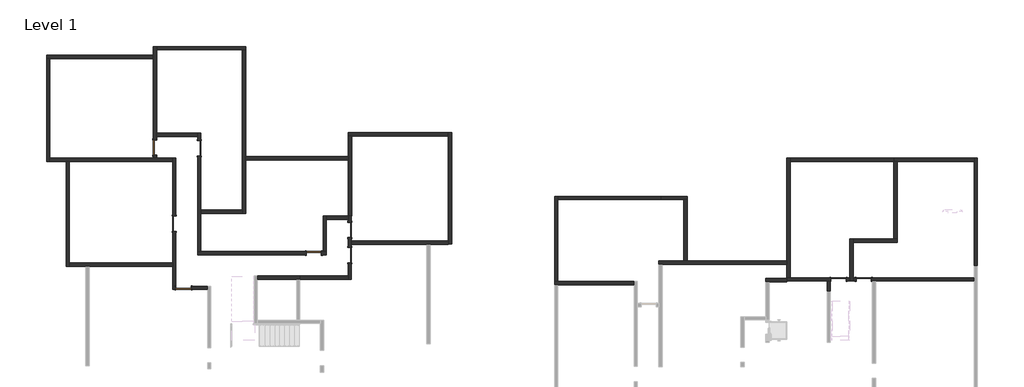
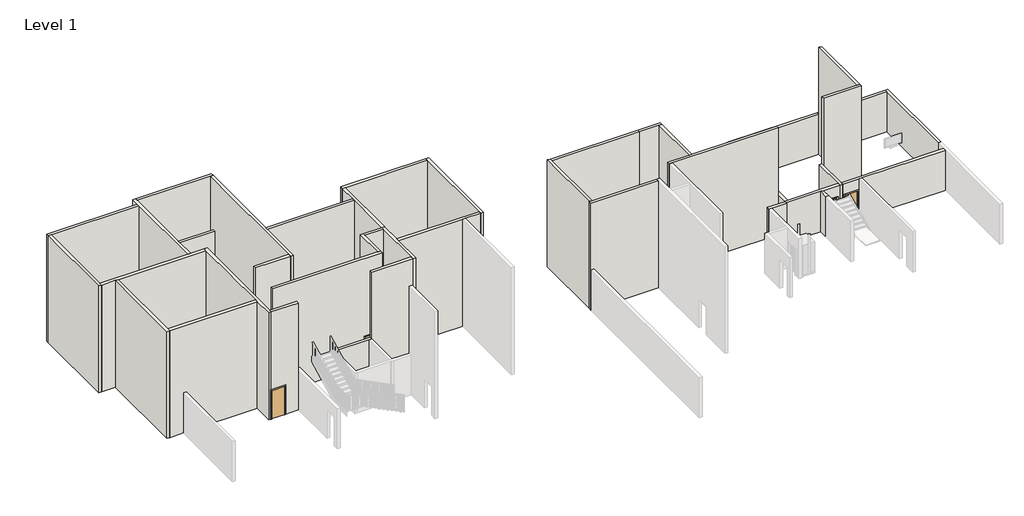
# One storey, part 2 of 3: 41 walls, 9 doors.
"""IFC4 building model written with IfcOpenShell, lengths in millimetres."""

import ifcopenshell
import ifcopenshell.guid

model = None  # the IFC model being written
_history = None  # IfcOwnerHistory: only IFC2X3 demands one
_inside = {}  # id of a spatial element -> (the spatial element, [elements in it])
_under = {}  # id of a project, library or spatial element -> (it, [spatial elements below it])
_declared = {}  # id of a project -> (the project, [libraries it declares])
_typed = {}  # id of a type object -> (the type object, [elements of that type])
_made_of = {}  # id of a material, layer set ... -> (it, [elements and type objects made of it])


def new_model(schema):
    """Start an empty IFC model of exactly this schema.

    Asked for "IFC4X3", IfcOpenShell would pick the latest addendum, in which some entities
    have other attributes; the version numbers below select the first issue.
    IFC2X3 requires an IfcOwnerHistory on every rooted entity: one is made here for all.
    """
    global model, _history
    if schema == "IFC4X3":
        model = ifcopenshell.file(schema_version=(4, 3, 0, 0))
    else:
        model = ifcopenshell.file(schema=schema)
    _inside.clear()
    _under.clear()
    _declared.clear()
    _typed.clear()
    _made_of.clear()
    _history = None
    if model.schema == "IFC2X3":
        org = make("IfcOrganization", Name="unknown")
        user = make(
            "IfcPersonAndOrganization",
            ThePerson=make("IfcPerson", FamilyName="unknown"),
            TheOrganization=org,
        )
        app = make(
            "IfcApplication",
            ApplicationDeveloper=org,
            Version="unknown",
            ApplicationFullName="unknown",
            ApplicationIdentifier="unknown",
        )
        _history = make(
            "IfcOwnerHistory",
            OwningUser=user,
            OwningApplication=app,
            ChangeAction="ADDED",
            CreationDate=0,
        )
    return model


def make(cls, **values):
    """One entity of the class cls with the attributes given. An attribute that is None is left unset."""
    return model.create_entity(
        cls, **{name: value for name, value in values.items() if value is not None}
    )


def rooted(cls, **values):
    """An entity with a GlobalId (a new one), such as an element, a storey or a relation."""
    return make(cls, GlobalId=ifcopenshell.guid.new(), OwnerHistory=_history, **values)


def si_unit(unit_type, name, prefix=None):
    """IfcSIUnit, for example si_unit("LENGTHUNIT", "METRE", prefix="MILLI")."""
    return make("IfcSIUnit", UnitType=unit_type, Prefix=prefix, Name=name)


def assignment(units):
    """IfcUnitAssignment: the units of a project."""
    return None if units is None else make("IfcUnitAssignment", Units=units)


def point(xyz):
    """IfcCartesianPoint."""
    return None if xyz is None else make("IfcCartesianPoint", Coordinates=xyz)


def direction(xyz):
    """IfcDirection."""
    return None if xyz is None else make("IfcDirection", DirectionRatios=xyz)


def frame(location, z_axis=None, x_axis=None):
    """IfcAxis2Placement3D, a coordinate frame: its origin and axes. An axis left out is left unset."""
    return make(
        "IfcAxis2Placement3D",
        Location=point(location),
        Axis=direction(z_axis),
        RefDirection=direction(x_axis),
    )


def origin():
    """The frame at (0, 0, 0) with its axes left unset."""
    return frame((0.0, 0.0, 0.0))


def origin_with_axes():
    """The frame at (0, 0, 0) with the z axis (0, 0, 1) and the x axis (1, 0, 0) written out."""
    return frame((0.0, 0.0, 0.0), z_axis=(0.0, 0.0, 1.0), x_axis=(1.0, 0.0, 0.0))


def place(relative_to, where):
    """IfcLocalPlacement: puts the frame where relative to a parent placement (None: the world)."""
    return make(
        "IfcLocalPlacement", PlacementRelTo=relative_to, RelativePlacement=where
    )


def context(
    kind, dimensions, precision=None, world=None, true_north=None, identifier=None
):
    """IfcGeometricRepresentationContext, for example the 3D "Model" context."""
    return make(
        "IfcGeometricRepresentationContext",
        ContextIdentifier=identifier,
        ContextType=kind,
        CoordinateSpaceDimension=dimensions,
        Precision=precision,
        WorldCoordinateSystem=world,
        TrueNorth=true_north,
    )


def project(units=None, contexts=None):
    """IfcProject with its units and contexts."""
    return rooted(
        "IfcProject",
        Name="project",
        RepresentationContexts=contexts,
        UnitsInContext=assignment(units),
    )


def spatial(cls, under=None, at=None, **own):
    """A site, building, storey or space (cls), placed at a placement, below another one or the project."""
    s = rooted(cls, ObjectPlacement=at, **own)
    if under is not None:
        _under.setdefault(under.id(), (under, []))[1].append(s)
    return s


def polyline(points):
    """IfcPolyline through the points."""
    return make("IfcPolyline", Points=[point(p) for p in points])


def outline(outer, holes=None, kind="AREA"):
    """IfcArbitraryClosedProfileDef: a profile drawn as a closed curve; with holes, ...WithVoids."""
    if holes is None:
        return make("IfcArbitraryClosedProfileDef", ProfileType=kind, OuterCurve=outer)
    return make(
        "IfcArbitraryProfileDefWithVoids",
        ProfileType=kind,
        OuterCurve=outer,
        InnerCurves=holes,
    )


def extrude(swept, where, along, depth):
    """IfcExtrudedAreaSolid: the profile swept, set in the frame where, extruded along a direction by depth."""
    return make(
        "IfcExtrudedAreaSolid",
        SweptArea=swept,
        Position=where,
        ExtrudedDirection=direction(along),
        Depth=depth,
    )


def faces_of(points, faces, orient=None, outer=None):
    """IfcFace entities. A face is a list of loops; a loop is a list of indices into points, from 0.

    orient and outer hold one flag for each loop. By default every Orientation is true, the
    first loop of a face is its IfcFaceOuterBound and the others are IfcFaceBound.
    """
    made = []
    for i, loops in enumerate(faces):
        bounds = []
        for j, loop in enumerate(loops):
            is_outer = j == 0 if outer is None else outer[i][j]
            bounds.append(
                make(
                    "IfcFaceOuterBound" if is_outer else "IfcFaceBound",
                    Bound=make("IfcPolyLoop", Polygon=[points[k] for k in loop]),
                    Orientation=True if orient is None else orient[i][j],
                )
            )
        made.append(make("IfcFace", Bounds=bounds))
    return made


def faceted_brep(points, faces, orient=None, outer=None, voids=None):
    """IfcFacetedBrep: a solid bounded by flat faces; with voids (closed shells), ...WithVoids."""
    shared = [point(p) for p in points]
    hull = make("IfcClosedShell", CfsFaces=faces_of(shared, faces, orient, outer))
    if voids is None:
        return make("IfcFacetedBrep", Outer=hull)
    return make(
        "IfcFacetedBrepWithVoids",
        Outer=hull,
        Voids=[
            make(cls, CfsFaces=faces_of(shared, fs, o, b)) for cls, fs, o, b in voids
        ],
    )


def shape(context_of_items, identifier, shape_type, items):
    """IfcShapeRepresentation: the items that make up one representation, for example the "Body"."""
    return make(
        "IfcShapeRepresentation",
        ContextOfItems=context_of_items,
        RepresentationIdentifier=identifier,
        RepresentationType=shape_type,
        Items=items,
    )


def source(mapping_origin, context_of_items, identifier, shape_type, items):
    """IfcRepresentationMap: a shape defined once, which mapped items show again and again."""
    return make(
        "IfcRepresentationMap",
        MappingOrigin=mapping_origin,
        MappedRepresentation=shape(context_of_items, identifier, shape_type, items),
    )


def transform(
    local_origin,
    x_axis=None,
    y_axis=None,
    z_axis=None,
    scale=None,
    scale2=None,
    scale3=None,
    uniform=True,
):
    """IfcCartesianTransformationOperator3D, or its non-uniform kind. x_axis, y_axis, z_axis: its Axis1, 2, 3."""
    if uniform:
        return make(
            "IfcCartesianTransformationOperator3D",
            Axis1=direction(x_axis),
            Axis2=direction(y_axis),
            LocalOrigin=point(local_origin),
            Scale=scale,
            Axis3=direction(z_axis),
        )
    return make(
        "IfcCartesianTransformationOperator3DnonUniform",
        Axis1=direction(x_axis),
        Axis2=direction(y_axis),
        LocalOrigin=point(local_origin),
        Scale=scale,
        Axis3=direction(z_axis),
        Scale2=scale2,
        Scale3=scale3,
    )


def mapped(mapping_source, mapping_target):
    """IfcMappedItem: shows the shape of a source again, moved by a transform."""
    return make(
        "IfcMappedItem", MappingSource=mapping_source, MappingTarget=mapping_target
    )


def made_of(thing, what):
    """Note that an element or type object is made of a material, layer set ...; save() writes the relation."""
    if what is not None:
        _made_of.setdefault(what.id(), (what, []))[1].append(thing)
    return thing


def element(
    cls,
    number,
    at=None,
    inside=None,
    cuts=None,
    type_object=None,
    material=None,
    context=None,
    identifier="Body",
    shape_type=None,
    held_by="IfcProductDefinitionShape",
    body=None,
    shapes=None,
    **own,
):
    """One element of the class cls, such as IfcWall. Its Tag is "e" and its number.

    at: its placement. inside: the storey or other place that contains it. cuts: it is an
    opening in that element (IfcRelVoidsElement). A single representation is given by context,
    identifier, shape_type and body (its items); several are given by shapes. held_by: the class
    of the entity that holds the representations. save() writes the other relations.
    """
    e = rooted(cls, Tag="e%d" % number, ObjectPlacement=at, **own)
    if body is not None:
        shapes = [shape(context, identifier, shape_type, body)]
    if shapes is not None:
        e.Representation = make(held_by, Representations=shapes)
    if inside is not None:
        _inside.setdefault(inside.id(), (inside, []))[1].append(e)
    if cuts is not None:
        rooted(
            "IfcRelVoidsElement", RelatingBuildingElement=cuts, RelatedOpeningElement=e
        )
    if type_object is not None:
        _typed.setdefault(type_object.id(), (type_object, []))[1].append(e)
    return made_of(e, material)


def aggregate(whole, parts):
    """IfcRelAggregates: a whole, such as a stair, and the parts it consists of."""
    return rooted("IfcRelAggregates", RelatingObject=whole, RelatedObjects=parts)


def save(model, path):
    """Write the relations noted so far, then the file.

    IfcRelAggregates (storeys below a building ...), IfcRelContainedInSpatialStructure (elements
    in a storey), IfcRelDefinesByType, IfcRelAssociatesMaterial and IfcRelDeclares: one each for
    every whole, place, type object, material and project.
    """
    for whole, parts in _under.values():
        aggregate(whole, parts)
    for where, things in _inside.values():
        rooted(
            "IfcRelContainedInSpatialStructure",
            RelatedElements=things,
            RelatingStructure=where,
        )
    for kind, things in _typed.values():
        rooted("IfcRelDefinesByType", RelatedObjects=things, RelatingType=kind)
    for what, things in _made_of.values():
        rooted("IfcRelAssociatesMaterial", RelatedObjects=things, RelatingMaterial=what)
    for by, libraries in _declared.values():
        rooted("IfcRelDeclares", RelatingContext=by, RelatedDefinitions=libraries)
    model.write(path)


def m_single_flush_0915_x_2134mm_727434cd(model_context):
    return source(origin(), model_context, "Body", "SweptSolid", [
        extrude(outline(polyline([(2210.0, -533.5), (0.0, -533.5), (0.0, -457.5), (2134.0, -457.5), (2134.0, 457.5), (0.0, 457.5), (0.0, 533.5), (2210.0, 533.5), (2210.0, -533.5)])), frame((0.0, -125.0, 0.0), z_axis=(0.0, 1.0, 0.0), x_axis=(0.0, 0.0, 1.0)), (0.0, 0.0, 1.0), 25.0),
        extrude(outline(polyline([(2210.0, 533.5), (2210.0, -533.5), (0.0, -533.5), (0.0, -457.5), (2134.0, -457.5), (2134.0, 457.5), (0.0, 457.5), (0.0, 533.5), (2210.0, 533.5)])), frame((0.0, 100.0, 0.0), z_axis=(0.0, 1.0, 0.0), x_axis=(0.0, 0.0, 1.0)), (0.0, 0.0, 1.0), 25.0),
        extrude(outline(polyline([(457.5, -49.0), (457.5, -100.0), (-457.5, -100.0), (-457.5, -49.0), (457.5, -49.0)])), origin_with_axes(), (0.0, 0.0, 1.0), 2134.0),
    ])


def m_single_flush_0915_x_2134mm_6a9e8738(model_context):
    return source(origin(), model_context, "Body", "SweptSolid", [
        extrude(outline(polyline([(2210.0, -533.5), (0.0, -533.5), (0.0, -457.5), (2134.0, -457.5), (2134.0, 457.5), (0.0, 457.5), (0.0, 533.5), (2210.0, 533.5), (2210.0, -533.5)])), frame((0.0, 100.0, 0.0), z_axis=(0.0, 1.0, 0.0), x_axis=(0.0, 0.0, 1.0)), (0.0, 0.0, 1.0), 25.0),
        extrude(outline(polyline([(2210.0, 533.5), (2210.0, -533.5), (0.0, -533.5), (0.0, -457.5), (2134.0, -457.5), (2134.0, 457.5), (0.0, 457.5), (0.0, 533.5), (2210.0, 533.5)])), frame((0.0, -125.0, 0.0), z_axis=(0.0, 1.0, 0.0), x_axis=(0.0, 0.0, 1.0)), (0.0, 0.0, 1.0), 25.0),
        extrude(outline(polyline([(457.5, 49.0), (-457.5, 49.0), (-457.5, 100.0), (457.5, 100.0), (457.5, 49.0)])), origin_with_axes(), (0.0, 0.0, 1.0), 2134.0),
    ])


model = new_model("IFC4")

# Units and contexts
model_context = context("Model", 3, world=origin())
ifc_project = project(units=[si_unit("LENGTHUNIT", "METRE", prefix="MILLI")], contexts=[model_context])

# Site, building, storey
site = spatial("IfcSite", under=ifc_project)
building = spatial("IfcBuilding", under=site)
storey = spatial("IfcBuildingStorey", under=building, Name="Level 1", Elevation=0.0)

# Doors
placement = place(None, origin())
m_single_flush_0915_x_2134mm_shape = m_single_flush_0915_x_2134mm_727434cd(model_context)
element("IfcDoor", 1, ObjectType="M_Single-Flush : 0915 x 2134mm", at=placement, inside=storey, context=model_context, shape_type="MappedRepresentation", body=[
    mapped(m_single_flush_0915_x_2134mm_shape, transform((23427.336337, 519.475628, 0.0), x_axis=(-1.0, 0.0, 0.0), y_axis=(0.0, -1.0, 0.0), z_axis=(0.0, 0.0, 1.0))),
])
element("IfcDoor", 2, ObjectType="M_Single-Flush : 0915 x 2134mm", at=placement, inside=storey, context=model_context, shape_type="MappedRepresentation", body=[
    mapped(m_single_flush_0915_x_2134mm_shape, transform((-7470.3551195, 1978.3372871, 0.0), x_axis=(0.0, 1.0, 0.0), y_axis=(-1.0, 0.0, 0.0), z_axis=(0.0, 0.0, 1.0))),
])
element("IfcDoor", 3, ObjectType="M_Single-Flush : 0915 x 2134mm", at=placement, inside=storey, context=model_context, shape_type="MappedRepresentation", body=[
    mapped(m_single_flush_0915_x_2134mm_shape, transform((-19189.8304233, 8462.8400285, 0.0), x_axis=(0.0, -1.0, 0.0), y_axis=(1.0, 0.0, 0.0), z_axis=(0.0, 0.0, 1.0))),
])
m_single_flush_0915_x_2134mm_2_shape = m_single_flush_0915_x_2134mm_6a9e8738(model_context)
element("IfcDoor", 4, ObjectType="M_Single-Flush : 0915 x 2134mm", at=placement, inside=storey, context=model_context, shape_type="MappedRepresentation", body=[
    mapped(m_single_flush_0915_x_2134mm_2_shape, transform((21912.336337, 519.475628, 0.0), x_axis=(1.0, 0.0, 0.0), y_axis=(0.0, 1.0, 0.0), z_axis=(0.0, 0.0, 1.0))),
])
element("IfcDoor", 5, ObjectType="M_Single-Flush : 0915 x 2134mm", at=placement, inside=storey, context=model_context, shape_type="MappedRepresentation", body=[
    mapped(m_single_flush_0915_x_2134mm_2_shape, transform((-17466.4741722, 12.8400285, 0.0), x_axis=(-1.0, 0.0, 0.0), y_axis=(0.0, -1.0, 0.0), z_axis=(0.0, 0.0, 1.0))),
])
element("IfcDoor", 6, ObjectType="M_Single-Flush : 0915 x 2134mm", at=placement, inside=storey, context=model_context, shape_type="MappedRepresentation", body=[
    mapped(m_single_flush_0915_x_2134mm_2_shape, transform((-18023.9741722, 3870.3400285, 0.0), x_axis=(0.0, 1.0, 0.0), y_axis=(-1.0, 0.0, 0.0), z_axis=(0.0, 0.0, 1.0))),
])
element("IfcDoor", 7, ObjectType="M_Single-Flush : 0915 x 2134mm", at=placement, inside=storey, context=model_context, shape_type="MappedRepresentation", body=[
    mapped(m_single_flush_0915_x_2134mm_2_shape, transform((-9627.8551195, 2100.8372871, 0.0), x_axis=(1.0, 0.0, 0.0), y_axis=(0.0, 1.0, 0.0), z_axis=(0.0, 0.0, 1.0))),
])
element("IfcDoor", 8, ObjectType="M_Single-Flush : 0915 x 2134mm", at=placement, inside=storey, context=model_context, shape_type="MappedRepresentation", body=[
    mapped(m_single_flush_0915_x_2134mm_2_shape, transform((-7470.3551195, 3488.3372871, 0.0), x_axis=(0.0, -1.0, 0.0), y_axis=(1.0, 0.0, 0.0), z_axis=(0.0, 0.0, 1.0))),
])
element("IfcDoor", 9, ObjectType="M_Single-Flush : 0915 x 2134mm", at=placement, inside=storey, context=model_context, shape_type="MappedRepresentation", body=[
    mapped(m_single_flush_0915_x_2134mm_2_shape, transform((-16523.9741722, 8415.3400285, 0.0), x_axis=(0.0, -1.0, 0.0), y_axis=(1.0, 0.0, 0.0), z_axis=(0.0, 0.0, 1.0))),
])

# Walls
element("IfcWall", 10, ObjectType="Generic - 200mm", at=placement, inside=storey, context=model_context, shape_type="Brep", body=[
    faceted_brep([(25249.836337, 7619.475628, 0.0), (25449.836337, 7619.475628, 0.0), (30068.3425199, 7619.475628, 0.0), (30068.3425199, 7619.475628, 3000.0), (25249.836337, 7619.475628, 3000.0), (25249.836337, 7819.475628, 0.0), (25249.836337, 7819.475628, 3000.0), (30068.3425199, 7819.475628, 3000.0), (30068.3425199, 7819.475628, 0.0)], [[[0, 1, 2, 3, 4]], [[5, 6, 7, 8]], [[2, 1, 0, 5, 8]], [[4, 3, 7, 6]], [[3, 2, 8, 7]], [[0, 4, 6, 5]]]),
])
element("IfcWall", 11, ObjectType="Generic - 200mm", at=placement, inside=storey, context=model_context, shape_type="Brep", body=[
    faceted_brep([(30068.3425199, 7819.475628, 0.0), (30068.3425199, 7619.475628, 0.0), (30068.3425199, 1319.475628, 0.0), (30068.3425199, 1319.475628, 3000.0), (30068.3425199, 7619.475628, 3000.0), (30068.3425199, 7819.475628, 3000.0), (30268.3425199, 7819.475628, 0.0), (30268.3425199, 7819.475628, 3000.0), (30268.3425199, 1319.475628, 3000.0), (30268.3425199, 1319.475628, 0.0), (30068.8612349, 1319.475628, 0.0), (30068.8612349, 1319.475628, 3000.0)], [[[0, 1, 2, 3, 4, 5]], [[6, 7, 8, 9]], [[2, 1, 0, 6, 9, 10]], [[3, 2, 10, 9, 8, 11]], [[5, 4, 3, 11, 8, 7]], [[0, 5, 7, 6]]]),
])
element("IfcWall", 12, ObjectType="Generic - 200mm", at=placement, inside=storey, context=model_context, shape_type="SweptSolid", body=[
    extrude(outline(polyline([(21429.836337, 419.475628), (21429.836337, -200.524372), (21229.836337, -200.524372), (21229.836337, 419.475628), (21429.836337, 419.475628)])), origin_with_axes(), (0.0, 0.0, 1.0), 3000.0),
])
element("IfcWall", 13, ObjectType="Generic - 200mm", at=placement, inside=storey, context=model_context, shape_type="SweptSolid", body=[
    extrude(outline(polyline([(25249.836337, 7619.475628), (19008.8612349, 7619.475628), (19008.8612349, 7819.475628), (25249.836337, 7819.475628), (25249.836337, 7619.475628)])), origin_with_axes(), (0.0, 0.0, 1.0), 3000.0),
])
element("IfcWall", 14, ObjectType="Generic - 200mm", at=placement, inside=storey, context=model_context, shape_type="Brep", body=[
    faceted_brep([(22788.8612349, 419.475628, 0.0), (22788.8612349, 619.475628, 0.0), (22788.8612349, 2754.475628, 0.0), (22788.8612349, 2954.475628, 0.0), (22788.8612349, 2954.475628, 3000.0), (22788.8612349, 619.475628, 3000.0), (22788.8612349, 419.475628, 3000.0), (22588.8612349, 419.475628, 0.0), (22588.8612349, 419.475628, 3000.0), (22588.8612349, 619.475628, 3000.0), (22588.8612349, 2954.475628, 3000.0), (22588.8612349, 2954.475628, 0.0), (22588.8612349, 619.475628, 0.0)], [[[0, 1, 2, 3, 4, 5, 6]], [[7, 8, 9, 10, 11, 12]], [[3, 2, 1, 0, 7, 12, 11]], [[6, 5, 4, 10, 9, 8]], [[0, 6, 8, 7]], [[4, 3, 11, 10]]]),
])
element("IfcWall", 15, ObjectType="Generic - 200mm", at=placement, inside=storey, context=model_context, shape_type="Brep", body=[
    faceted_brep([(18808.8612349, 7819.475628, 0.0), (18808.8612349, 1619.475628, 0.0), (18808.8612349, 1419.475628, 0.0), (18808.8612349, 619.475628, 0.0), (18808.8612349, 619.475628, 3000.0), (18808.8612349, 7819.475628, 3000.0), (19008.8612349, 7819.475628, 0.0), (19008.8612349, 7819.475628, 3000.0), (19008.8612349, 7619.475628, 3000.0), (19008.8612349, 619.475628, 3000.0), (19008.8612349, 619.475628, 0.0), (19008.8612349, 7619.475628, 0.0)], [[[0, 1, 2, 3, 4, 5]], [[6, 7, 8, 9, 10, 11]], [[3, 2, 1, 0, 6, 11, 10]], [[5, 4, 9, 8, 7]], [[4, 3, 10, 9]], [[0, 5, 7, 6]]]),
])
element("IfcWall", 16, ObjectType="Generic - 200mm", at=placement, inside=storey, context=model_context, shape_type="Brep", body=[
    faceted_brep([(30068.8612349, 419.475628, 3000.0), (24148.8612349, 419.475628, 3000.0), (23948.8612349, 419.475628, 3000.0), (22788.8612349, 419.475628, 3000.0), (22788.8612349, 419.475628, 0.0), (22969.836337, 419.475628, 0.0), (22969.836337, 419.475628, 2134.0), (23884.836337, 419.475628, 2134.0), (23884.836337, 419.475628, 0.0), (23948.8612349, 419.475628, 0.0), (24148.8612349, 419.475628, 0.0), (30068.8612349, 419.475628, 0.0), (22788.8612349, 619.475628, 3000.0), (30068.8612349, 619.475628, 3000.0), (30068.8612349, 619.475628, 0.0), (23884.836337, 619.475628, 0.0), (23884.836337, 619.475628, 2134.0), (22969.836337, 619.475628, 2134.0), (22969.836337, 619.475628, 0.0), (22788.8612349, 619.475628, 0.0)], [[[0, 1, 2, 3, 4, 5, 6, 7, 8, 9, 10, 11]], [[12, 13, 14, 15, 16, 17, 18, 19]], [[14, 11, 10, 9, 8, 15]], [[4, 19, 18, 5]], [[3, 2, 1, 0, 13, 12]], [[0, 11, 14, 13]], [[4, 3, 12, 19]], [[17, 6, 5, 18]], [[7, 16, 15, 8]], [[16, 7, 6, 17]]]),
])
element("IfcWall", 17, ObjectType="Generic - 200mm", at=placement, inside=storey, context=model_context, shape_type="Brep", body=[
    faceted_brep([(18808.8612349, 579.475628, 0.0), (17550.6041014, 579.475628, 0.0), (17550.6041014, 579.475628, 3000.0), (18808.8612349, 579.475628, 3000.0), (18808.8612349, 379.475628, 0.0), (18808.8612349, 379.475628, 3000.0), (17750.6041014, 379.475628, 3000.0), (17550.6041014, 379.475628, 3000.0), (17550.6041014, 379.475628, 0.0), (17750.6041014, 379.475628, 0.0), (18808.8612349, 419.475628, 0.0), (18808.8612349, 419.475628, 3000.0)], [[[0, 1, 2, 3]], [[4, 5, 6, 7, 8, 9]], [[1, 0, 10, 4, 9, 8]], [[3, 2, 7, 6, 5, 11]], [[0, 3, 11, 5, 4, 10]], [[2, 1, 8, 7]]]),
])
element("IfcWall", 18, ObjectType="Generic - 200mm", at=placement, inside=storey, context=model_context, shape_type="Brep", body=[
    faceted_brep([(18808.8612349, 619.475628, 3000.0), (19008.8612349, 619.475628, 3000.0), (22588.8612349, 619.475628, 3000.0), (22588.8612349, 619.475628, 0.0), (22369.836337, 619.475628, 0.0), (22369.836337, 619.475628, 2134.0), (21454.836337, 619.475628, 2134.0), (21454.836337, 619.475628, 0.0), (19008.8612349, 619.475628, 0.0), (18808.8612349, 619.475628, 0.0), (22588.8612349, 419.475628, 3000.0), (21429.836337, 419.475628, 3000.0), (21229.836337, 419.475628, 3000.0), (18808.8612349, 419.475628, 3000.0), (18808.8612349, 419.475628, 0.0), (21229.836337, 419.475628, 0.0), (21429.836337, 419.475628, 0.0), (21454.836337, 419.475628, 0.0), (21454.836337, 419.475628, 2134.0), (22369.836337, 419.475628, 2134.0), (22369.836337, 419.475628, 0.0), (22588.8612349, 419.475628, 0.0), (18808.8612349, 579.475628, 0.0), (18808.8612349, 579.475628, 3000.0)], [[[0, 1, 2, 3, 4, 5, 6, 7, 8, 9]], [[10, 11, 12, 13, 14, 15, 16, 17, 18, 19, 20, 21]], [[3, 21, 20, 4]], [[14, 22, 9, 8, 7, 17, 16, 15]], [[2, 1, 0, 23, 13, 12, 11, 10]], [[0, 9, 22, 14, 13, 23]], [[3, 2, 10, 21]], [[19, 5, 4, 20]], [[6, 18, 17, 7]], [[18, 6, 5, 19]]]),
])
element("IfcWall", 19, ObjectType="Generic - 200mm", at=placement, inside=storey, context=model_context, shape_type="Brep", body=[
    faceted_brep([(22788.8612349, 2754.475628, 0.0), (25449.836337, 2754.475628, 0.0), (25449.836337, 2754.475628, 8000.0), (22788.8612349, 2754.475628, 8000.0), (22788.8612349, 2954.475628, 0.0), (22788.8612349, 2954.475628, 3000.0), (22788.8612349, 2954.475628, 8000.0), (25249.836337, 2954.475628, 8000.0), (25449.836337, 2954.475628, 8000.0), (25449.836337, 2954.475628, 0.0), (25249.836337, 2954.475628, 0.0)], [[[0, 1, 2, 3]], [[4, 5, 6, 7, 8, 9, 10]], [[1, 0, 4, 10, 9]], [[3, 2, 8, 7, 6]], [[2, 1, 9, 8]], [[0, 3, 6, 5, 4]]]),
])
element("IfcWall", 20, ObjectType="Generic - 200mm", at=placement, inside=storey, context=model_context, shape_type="Brep", body=[
    faceted_brep([(25449.836337, 2954.475628, 0.0), (25449.836337, 7619.475628, 0.0), (25449.836337, 7619.475628, 8000.0), (25449.836337, 2954.475628, 8000.0), (25249.836337, 2954.475628, 0.0), (25249.836337, 2954.475628, 8000.0), (25249.836337, 7619.475628, 8000.0), (25249.836337, 7619.475628, 3000.0), (25249.836337, 7619.475628, 0.0)], [[[0, 1, 2, 3]], [[4, 5, 6, 7, 8]], [[1, 0, 4, 8]], [[3, 2, 6, 5]], [[0, 3, 5, 4]], [[2, 1, 8, 7, 6]]]),
])
element("IfcWall", 21, ObjectType="Generic - 200mm", at=placement, inside=storey, context=model_context, shape_type="Brep", body=[
    faceted_brep([(-10469.8304233, 720.8372871, 0.0), (-13026.101437, 720.8372871, 0.0), (-13026.101437, 720.8372871, 3000.0), (-10469.8304233, 720.8372871, 3000.0), (-10469.8304233, 520.8372871, 0.0), (-10469.8304233, 520.8372871, 3000.0), (-10669.8304233, 520.8372871, 3000.0), (-13026.101437, 520.8372871, 3000.0), (-13026.101437, 520.8372871, 0.0), (-10669.8304233, 520.8372871, 0.0)], [[[0, 1, 2, 3]], [[4, 5, 6, 7, 8, 9]], [[1, 0, 4, 9, 8]], [[3, 2, 7, 6, 5]], [[2, 1, 8, 7]], [[0, 3, 5, 4]]]),
])
element("IfcWall", 22, ObjectType="Generic - 200mm", at=placement, inside=storey, context=model_context, shape_type="Brep", body=[
    faceted_brep([(-19089.8304233, 7812.8400285, 0.0), (-19089.8304233, 8005.3400285, 0.0), (-19089.8304233, 8005.3400285, 2134.0), (-19089.8304233, 8920.3400285, 2134.0), (-19089.8304233, 8920.3400285, 0.0), (-19089.8304233, 9112.8400285, 0.0), (-19089.8304233, 9312.8400285, 0.0), (-19089.8304233, 14340.8372871, 0.0), (-19089.8304233, 14540.8372871, 0.0), (-19089.8304233, 14540.8372871, 8000.0), (-19089.8304233, 14340.8372871, 8000.0), (-19089.8304233, 9312.8400285, 8000.0), (-19089.8304233, 9112.8400285, 8000.0), (-19089.8304233, 7812.8400285, 8000.0), (-19289.8304233, 8005.3400285, 2134.0), (-19289.8304233, 8005.3400285, 0.0), (-19289.8304233, 7812.8400285, 0.0), (-19289.8304233, 7812.8400285, 8000.0), (-19289.8304233, 13812.8400285, 8000.0), (-19289.8304233, 14012.8400285, 8000.0), (-19289.8304233, 14540.8372871, 8000.0), (-19289.8304233, 14540.8372871, 0.0), (-19289.8304233, 14012.8400285, 0.0), (-19289.8304233, 13812.8400285, 0.0), (-19289.8304233, 8920.3400285, 0.0), (-19289.8304233, 8920.3400285, 2134.0)], [[[0, 1, 2, 3, 4, 5, 6, 7, 8, 9, 10, 11, 12, 13]], [[14, 15, 16, 17, 18, 19, 20, 21, 22, 23, 24, 25]], [[16, 15, 1, 0]], [[24, 23, 22, 21, 8, 7, 6, 5, 4]], [[13, 12, 11, 10, 9, 20, 19, 18, 17]], [[9, 8, 21, 20]], [[0, 13, 17, 16]], [[2, 1, 15, 14]], [[3, 2, 14, 25]], [[4, 3, 25, 24]]]),
])
element("IfcWall", 23, ObjectType="Generic - 200mm", at=placement, inside=storey, context=model_context, shape_type="Brep", body=[
    faceted_brep([(9628.8612349, 399.9901881, 0.0), (5043.716007, 399.9901881, 0.0), (4843.716007, 399.9901881, 0.0), (4843.716007, 399.9901881, 8000.0), (5043.716007, 399.9901881, 8000.0), (9628.8612349, 399.9901881, 8000.0), (9628.8612349, 199.9901881, 0.0), (9628.8612349, 199.9901881, 8000.0), (4843.716007, 199.9901881, 8000.0), (4843.716007, 199.9901881, 3000.0), (4843.716007, 199.9901881, 0.0), (5043.716007, 199.9901881, 0.0)], [[[0, 1, 2, 3, 4, 5]], [[6, 7, 8, 9, 10, 11]], [[2, 1, 0, 6, 11, 10]], [[5, 4, 3, 8, 7]], [[0, 5, 7, 6]], [[2, 10, 9, 8, 3]]]),
])
element("IfcWall", 24, ObjectType="Generic - 200mm", at=placement, inside=storey, context=model_context, shape_type="Brep", body=[
    faceted_brep([(-13726.101437, 14540.8372871, 0.0), (-19089.8304233, 14540.8372871, 0.0), (-19089.8304233, 14540.8372871, 8000.0), (-13726.101437, 14540.8372871, 8000.0), (-13726.101437, 14340.8372871, 0.0), (-13726.101437, 14340.8372871, 8000.0), (-13926.101437, 14340.8372871, 8000.0), (-19089.8304233, 14340.8372871, 8000.0), (-19089.8304233, 14340.8372871, 0.0), (-13926.101437, 14340.8372871, 0.0)], [[[0, 1, 2, 3]], [[4, 5, 6, 7, 8, 9]], [[1, 0, 4, 9, 8]], [[3, 2, 7, 6, 5]], [[2, 1, 8, 7]], [[0, 3, 5, 4]]]),
])
element("IfcWall", 25, ObjectType="Generic - 200mm", at=placement, inside=storey, context=model_context, shape_type="Brep", body=[
    faceted_brep([(-25701.4369496, 13812.8400285, 0.0), (-25701.4369496, 7612.8400285, 0.0), (-25701.4369496, 7612.8400285, 8000.0), (-25701.4369496, 13812.8400285, 8000.0), (-25501.4369496, 13812.8400285, 0.0), (-25501.4369496, 13812.8400285, 8000.0), (-25501.4369496, 7812.8400285, 8000.0), (-25501.4369496, 7612.8400285, 8000.0), (-25501.4369496, 7612.8400285, 0.0), (-25501.4369496, 7812.8400285, 0.0)], [[[0, 1, 2, 3]], [[4, 5, 6, 7, 8, 9]], [[1, 0, 4, 9, 8]], [[3, 2, 7, 6, 5]], [[2, 1, 8, 7]], [[0, 3, 5, 4]]]),
])
element("IfcWall", 26, ObjectType="Generic - 200mm", at=placement, inside=storey, context=model_context, shape_type="Brep", body=[
    faceted_brep([(-25501.4369496, 7612.8400285, 0.0), (-24523.9741722, 7612.8400285, 0.0), (-24323.9741722, 7612.8400285, 0.0), (-18123.9741722, 7612.8400285, 0.0), (-18123.9741722, 7612.8400285, 8000.0), (-24323.9741722, 7612.8400285, 8000.0), (-24523.9741722, 7612.8400285, 8000.0), (-25501.4369496, 7612.8400285, 8000.0), (-25501.4369496, 7812.8400285, 0.0), (-25501.4369496, 7812.8400285, 8000.0), (-19289.8304233, 7812.8400285, 8000.0), (-19089.8304233, 7812.8400285, 8000.0), (-18123.9741722, 7812.8400285, 8000.0), (-18123.9741722, 7812.8400285, 0.0), (-19089.8304233, 7812.8400285, 0.0), (-19289.8304233, 7812.8400285, 0.0)], [[[0, 1, 2, 3, 4, 5, 6, 7]], [[8, 9, 10, 11, 12, 13, 14, 15]], [[3, 2, 1, 0, 8, 15, 14, 13]], [[7, 6, 5, 4, 12, 11, 10, 9]], [[0, 7, 9, 8]], [[4, 3, 13, 12]]]),
])
element("IfcWall", 27, ObjectType="Generic - 200mm", at=placement, inside=storey, context=model_context, shape_type="Brep", body=[
    faceted_brep([(-19289.8304233, 14012.8400285, 0.0), (-25701.4369496, 14012.8400285, 0.0), (-25701.4369496, 14012.8400285, 8000.0), (-19289.8304233, 14012.8400285, 8000.0), (-19289.8304233, 13812.8400285, 0.0), (-19289.8304233, 13812.8400285, 8000.0), (-25501.4369496, 13812.8400285, 8000.0), (-25701.4369496, 13812.8400285, 8000.0), (-25701.4369496, 13812.8400285, 0.0), (-25501.4369496, 13812.8400285, 0.0)], [[[0, 1, 2, 3]], [[4, 5, 6, 7, 8, 9]], [[1, 0, 4, 9, 8]], [[3, 2, 7, 6, 5]], [[2, 1, 8, 7]], [[0, 3, 5, 4]]]),
])
element("IfcWall", 28, ObjectType="Generic - 200mm", at=placement, inside=storey, context=model_context, shape_type="Brep", body=[
    faceted_brep([(-24523.9741722, 7612.8400285, 0.0), (-24523.9741722, 1312.8400285, 0.0), (-24523.9741722, 1312.8400285, 8000.0), (-24523.9741722, 7612.8400285, 8000.0), (-24323.9741722, 7612.8400285, 0.0), (-24323.9741722, 7612.8400285, 8000.0), (-24323.9741722, 1512.8400285, 8000.0), (-24323.9741722, 1312.8400285, 8000.0), (-24323.9741722, 1312.8400285, 0.0), (-24323.9741722, 1512.8400285, 0.0)], [[[0, 1, 2, 3]], [[4, 5, 6, 7, 8, 9]], [[1, 0, 4, 9, 8]], [[3, 2, 7, 6, 5]], [[0, 3, 5, 4]], [[2, 1, 8, 7]]]),
])
element("IfcWall", 29, ObjectType="Generic - 200mm", at=placement, inside=storey, context=model_context, shape_type="Brep", body=[
    faceted_brep([(-24323.9741722, 1312.8400285, 0.0), (-23346.5113948, 1312.8400285, 0.0), (-23146.5113948, 1312.8400285, 0.0), (-18123.9741722, 1312.8400285, 0.0), (-18123.9741722, 1312.8400285, 8000.0), (-24323.9741722, 1312.8400285, 8000.0), (-24323.9741722, 1512.8400285, 0.0), (-24323.9741722, 1512.8400285, 8000.0), (-18123.9741722, 1512.8400285, 8000.0), (-18123.9741722, 1512.8400285, 0.0)], [[[0, 1, 2, 3, 4, 5]], [[6, 7, 8, 9]], [[3, 2, 1, 0, 6, 9]], [[5, 4, 8, 7]], [[0, 5, 7, 6]], [[4, 3, 9, 8]]]),
])
element("IfcWall", 30, ObjectType="Generic - 200mm", at=placement, inside=storey, context=model_context, shape_type="Brep", body=[
    faceted_brep([(-19089.8304233, 9112.8400285, 0.0), (-16623.9741722, 9112.8400285, 0.0), (-16623.9741722, 9112.8400285, 2134.0), (-16623.9741722, 9112.8400285, 8000.0), (-19089.8304233, 9112.8400285, 8000.0), (-19089.8304233, 9312.8400285, 0.0), (-19089.8304233, 9312.8400285, 8000.0), (-16623.9741722, 9312.8400285, 8000.0), (-16623.9741722, 9312.8400285, 3000.0), (-16623.9741722, 9312.8400285, 0.0)], [[[0, 1, 2, 3, 4]], [[5, 6, 7, 8, 9]], [[1, 0, 5, 9]], [[4, 3, 7, 6]], [[0, 4, 6, 5]], [[3, 2, 1, 9, 8, 7]]]),
])
element("IfcWall", 31, ObjectType="Generic - 200mm", at=placement, inside=storey, context=model_context, shape_type="Brep", body=[
    faceted_brep([(-18123.9741722, 7812.8400285, 0.0), (-18123.9741722, 7612.8400285, 0.0), (-18123.9741722, 4327.8400285, 0.0), (-18123.9741722, 4327.8400285, 2134.0), (-18123.9741722, 3412.8400285, 2134.0), (-18123.9741722, 3412.8400285, 0.0), (-18123.9741722, 1512.8400285, 0.0), (-18123.9741722, 1312.8400285, 0.0), (-18123.9741722, -87.1599715, 0.0), (-18123.9741722, -87.1599715, 8000.0), (-18123.9741722, 1312.8400285, 8000.0), (-18123.9741722, 1512.8400285, 8000.0), (-18123.9741722, 7612.8400285, 8000.0), (-18123.9741722, 7812.8400285, 8000.0), (-17923.9741722, 4327.8400285, 2134.0), (-17923.9741722, 4327.8400285, 0.0), (-17923.9741722, 7812.8400285, 0.0), (-17923.9741722, 7812.8400285, 8000.0), (-17923.9741722, 112.8400285, 8000.0), (-17923.9741722, -87.1599715, 8000.0), (-17923.9741722, -87.1599715, 2134.0), (-17923.9741722, -87.1599715, 0.0), (-17923.9741722, 3412.8400285, 0.0), (-17923.9741722, 3412.8400285, 2134.0)], [[[0, 1, 2, 3, 4, 5, 6, 7, 8, 9, 10, 11, 12, 13]], [[14, 15, 16, 17, 18, 19, 20, 21, 22, 23]], [[22, 21, 8, 7, 6, 5]], [[16, 15, 2, 1, 0]], [[13, 12, 11, 10, 9, 19, 18, 17]], [[0, 13, 17, 16]], [[9, 8, 21, 20, 19]], [[3, 2, 15, 14]], [[4, 3, 14, 23]], [[5, 4, 23, 22]]]),
])
element("IfcWall", 32, ObjectType="Generic - 200mm", at=placement, inside=storey, context=model_context, shape_type="Brep", body=[
    faceted_brep([(-16013.9741722, -87.1599715, 8000.0), (-17923.9741722, -87.1599715, 8000.0), (-17923.9741722, -87.1599715, 2134.0), (-17008.9741722, -87.1599715, 2134.0), (-17008.9741722, -87.1599715, 0.0), (-16013.9741722, -87.1599715, 0.0), (-17923.9741722, 112.8400285, 8000.0), (-16013.9741722, 112.8400285, 8000.0), (-16013.9741722, 112.8400285, 3000.0), (-16013.9741722, 112.8400285, 0.0), (-17008.9741722, 112.8400285, 0.0), (-17008.9741722, 112.8400285, 2134.0), (-17923.9741722, 112.8400285, 2134.0)], [[[0, 1, 2, 3, 4, 5]], [[6, 7, 8, 9, 10, 11, 12]], [[9, 5, 4, 10]], [[1, 0, 7, 6]], [[1, 6, 12, 2]], [[0, 5, 9, 8, 7]], [[11, 3, 2, 12]], [[3, 11, 10, 4]]]),
])
element("IfcWall", 33, ObjectType="Generic - 200mm", at=placement, inside=storey, context=model_context, shape_type="Brep", body=[
    faceted_brep([(-16423.9741722, 2200.8372871, 0.0), (-16423.9741722, 4500.8372871, 0.0), (-16423.9741722, 4700.8372871, 0.0), (-16423.9741722, 7957.8400285, 0.0), (-16423.9741722, 7957.8400285, 2134.0), (-16423.9741722, 8872.8400285, 2134.0), (-16423.9741722, 8872.8400285, 0.0), (-16423.9741722, 9312.8400285, 0.0), (-16423.9741722, 9312.8400285, 3000.0), (-16423.9741722, 2200.8372871, 3000.0), (-16623.9741722, 7957.8400285, 2134.0), (-16623.9741722, 7957.8400285, 0.0), (-16623.9741722, 2200.8372871, 0.0), (-16623.9741722, 2200.8372871, 3000.0), (-16623.9741722, 9312.8400285, 3000.0), (-16623.9741722, 9312.8400285, 0.0), (-16623.9741722, 9112.8400285, 0.0), (-16623.9741722, 8872.8400285, 0.0), (-16623.9741722, 8872.8400285, 2134.0)], [[[0, 1, 2, 3, 4, 5, 6, 7, 8, 9]], [[10, 11, 12, 13, 14, 15, 16, 17, 18]], [[12, 11, 3, 2, 1, 0]], [[17, 16, 15, 7, 6]], [[9, 8, 14, 13]], [[0, 9, 13, 12]], [[8, 7, 15, 14]], [[4, 3, 11, 10]], [[5, 4, 10, 18]], [[6, 5, 18, 17]]]),
])
element("IfcWall", 34, ObjectType="Generic - 200mm", at=placement, inside=storey, context=model_context, shape_type="SweptSolid", body=[
    extrude(outline(polyline([(-13726.101437, 7900.8372871), (-7565.3629108, 7900.8372871), (-7565.3629108, 7700.8372871), (-13726.101437, 7700.8372871), (-13726.101437, 7900.8372871)])), origin_with_axes(), (0.0, 0.0, 1.0), 8000.0),
])
element("IfcWall", 35, ObjectType="Generic - 200mm", at=placement, inside=storey, context=model_context, shape_type="Brep", body=[
    faceted_brep([(-9170.3551195, 2000.8372871, 2134.0), (-9170.3551195, 2000.8372871, 0.0), (-8870.3551195, 2000.8372871, 0.0), (-8870.3551195, 2000.8372871, 8000.0), (-16623.9741722, 2000.8372871, 8000.0), (-16623.9741722, 2000.8372871, 0.0), (-10085.3551195, 2000.8372871, 0.0), (-10085.3551195, 2000.8372871, 2134.0), (-8870.3551195, 2200.8372871, 0.0), (-9070.3551195, 2200.8372871, 0.0), (-9170.3551195, 2200.8372871, 0.0), (-9170.3551195, 2200.8372871, 2134.0), (-10085.3551195, 2200.8372871, 2134.0), (-10085.3551195, 2200.8372871, 0.0), (-16423.9741722, 2200.8372871, 0.0), (-16623.9741722, 2200.8372871, 0.0), (-16623.9741722, 2200.8372871, 3000.0), (-16623.9741722, 2200.8372871, 8000.0), (-9070.3551195, 2200.8372871, 8000.0), (-8870.3551195, 2200.8372871, 8000.0)], [[[0, 1, 2, 3, 4, 5, 6, 7]], [[8, 9, 10, 11, 12, 13, 14, 15, 16, 17, 18, 19]], [[6, 5, 15, 14, 13]], [[2, 1, 10, 9, 8]], [[4, 3, 19, 18, 17]], [[5, 4, 17, 16, 15]], [[3, 2, 8, 19]], [[11, 10, 1, 0]], [[12, 11, 0, 7]], [[13, 12, 7, 6]]]),
])
element("IfcWall", 36, ObjectType="Generic - 200mm", at=placement, inside=storey, context=model_context, shape_type="Brep", body=[
    faceted_brep([(-7570.3551195, 720.8372871, 0.0), (-10469.8304233, 720.8372871, 0.0), (-10469.8304233, 720.8372871, 3000.0), (-10469.8304233, 720.8372871, 8000.0), (-7570.3551195, 720.8372871, 8000.0), (-7570.3551195, 520.8372871, 0.0), (-7570.3551195, 520.8372871, 8000.0), (-10469.8304233, 520.8372871, 8000.0), (-10469.8304233, 520.8372871, 3000.0), (-10469.8304233, 520.8372871, 0.0)], [[[0, 1, 2, 3, 4]], [[5, 6, 7, 8, 9]], [[1, 0, 5, 9]], [[4, 3, 7, 6]], [[3, 2, 1, 9, 8, 7]], [[0, 4, 6, 5]]]),
])
element("IfcWall", 37, ObjectType="Generic - 200mm", at=placement, inside=storey, context=model_context, shape_type="Brep", body=[
    faceted_brep([(-1550.3449834, 9360.8372871, 0.0), (-1550.3449834, 9160.8372871, 0.0), (-1550.3449834, 2835.8372871, 0.0), (-1550.3449834, 2640.8372871, 0.0), (-1550.3449834, 2640.8372871, 8000.0), (-1550.3449834, 2835.8372871, 8000.0), (-1550.3449834, 9160.8372871, 8000.0), (-1550.3449834, 9360.8372871, 8000.0), (-1350.3449834, 9360.8372871, 0.0), (-1350.3449834, 9360.8372871, 8000.0), (-1350.3449834, 2640.8372871, 8000.0), (-1350.3449834, 2640.8372871, 0.0)], [[[0, 1, 2, 3, 4, 5, 6, 7]], [[8, 9, 10, 11]], [[3, 2, 1, 0, 8, 11]], [[4, 3, 11, 10]], [[7, 6, 5, 4, 10, 9]], [[0, 7, 9, 8]]]),
])
element("IfcWall", 38, ObjectType="Generic - 200mm", at=placement, inside=storey, context=model_context, shape_type="Brep", body=[
    faceted_brep([(11108.8612349, 1419.475628, 0.0), (11308.8612349, 1419.475628, 0.0), (18808.8612349, 1419.475628, 0.0), (18808.8612349, 1419.475628, 8000.0), (11308.8612349, 1419.475628, 8000.0), (11108.8612349, 1419.475628, 8000.0), (11108.8612349, 1619.475628, 0.0), (11108.8612349, 1619.475628, 8000.0), (12613.8612349, 1619.475628, 8000.0), (12813.8612349, 1619.475628, 8000.0), (18808.8612349, 1619.475628, 8000.0), (18808.8612349, 1619.475628, 0.0), (12813.8612349, 1619.475628, 0.0), (12613.8612349, 1619.475628, 0.0)], [[[0, 1, 2, 3, 4, 5]], [[6, 7, 8, 9, 10, 11, 12, 13]], [[2, 1, 0, 6, 13, 12, 11]], [[5, 4, 3, 10, 9, 8, 7]], [[3, 2, 11, 10]], [[0, 5, 7, 6]]]),
])
element("IfcWall", 39, ObjectType="Generic - 200mm", at=placement, inside=storey, context=model_context, shape_type="Brep", body=[
    faceted_brep([(5043.716007, 399.9901881, 0.0), (5043.716007, 5319.475628, 0.0), (5043.716007, 5519.475628, 0.0), (5043.716007, 5519.475628, 8000.0), (5043.716007, 5319.475628, 8000.0), (5043.716007, 399.9901881, 8000.0), (4843.716007, 399.9901881, 0.0), (4843.716007, 399.9901881, 8000.0), (4843.716007, 5519.475628, 8000.0), (4843.716007, 5519.475628, 0.0)], [[[0, 1, 2, 3, 4, 5]], [[6, 7, 8, 9]], [[2, 1, 0, 6, 9]], [[5, 4, 3, 8, 7]], [[0, 5, 7, 6]], [[3, 2, 9, 8]]]),
])
element("IfcWall", 40, ObjectType="Generic - 200mm", at=placement, inside=storey, context=model_context, shape_type="SweptSolid", body=[
    extrude(outline(polyline([(5043.716007, 5519.475628), (11228.8612349, 5519.475628), (11228.8612349, 5319.475628), (5043.716007, 5319.475628), (5043.716007, 5519.475628)])), origin_with_axes(), (0.0, 0.0, 1.0), 8000.0),
])
element("IfcWall", 41, ObjectType="Generic - 200mm", at=placement, inside=storey, context=model_context, shape_type="Brep", body=[
    faceted_brep([(-13926.101437, 14340.8372871, 0.0), (-13926.101437, 4700.8372871, 0.0), (-13926.101437, 4500.8372871, 0.0), (-13926.101437, 4500.8372871, 8000.0), (-13926.101437, 4700.8372871, 8000.0), (-13926.101437, 14340.8372871, 8000.0), (-13726.101437, 14340.8372871, 0.0), (-13726.101437, 14340.8372871, 8000.0), (-13726.101437, 7900.8372871, 8000.0), (-13726.101437, 7700.8372871, 8000.0), (-13726.101437, 4500.8372871, 8000.0), (-13726.101437, 4500.8372871, 0.0), (-13726.101437, 7700.8372871, 0.0), (-13726.101437, 7900.8372871, 0.0)], [[[0, 1, 2, 3, 4, 5]], [[6, 7, 8, 9, 10, 11, 12, 13]], [[2, 1, 0, 6, 13, 12, 11]], [[5, 4, 3, 10, 9, 8, 7]], [[3, 2, 11, 10]], [[0, 5, 7, 6]]]),
])
element("IfcWall", 42, ObjectType="Generic - 200mm", at=placement, inside=storey, context=model_context, shape_type="SweptSolid", body=[
    extrude(outline(polyline([(-16423.9741722, 4700.8372871), (-13926.101437, 4700.8372871), (-13926.101437, 4500.8372871), (-16423.9741722, 4500.8372871), (-16423.9741722, 4700.8372871)])), origin_with_axes(), (0.0, 0.0, 1.0), 8000.0),
])
element("IfcWall", 43, ObjectType="Generic - 200mm", at=placement, inside=storey, context=model_context, shape_type="Brep", body=[
    faceted_brep([(-7370.3551195, 2435.8372871, 2134.0), (-7370.3551195, 2435.8372871, 0.0), (-7370.3551195, 2635.8372871, 0.0), (-7370.3551195, 2835.8372871, 0.0), (-7370.3551195, 3030.8372871, 0.0), (-7370.3551195, 3030.8372871, 2134.0), (-7370.3551195, 3945.8372871, 2134.0), (-7370.3551195, 3945.8372871, 0.0), (-7370.3551195, 4340.8372871, 0.0), (-7370.3551195, 4340.8372871, 8000.0), (-7370.3551195, 2835.8372871, 8000.0), (-7370.3551195, 2635.8372871, 8000.0), (-7370.3551195, 520.8372871, 8000.0), (-7370.3551195, 520.8372871, 0.0), (-7370.3551195, 1520.8372871, 0.0), (-7370.3551195, 1520.8372871, 2134.0), (-7570.3551195, 3030.8372871, 0.0), (-7570.3551195, 2435.8372871, 0.0), (-7570.3551195, 2435.8372871, 2134.0), (-7570.3551195, 1520.8372871, 2134.0), (-7570.3551195, 1520.8372871, 0.0), (-7570.3551195, 720.8372871, 0.0), (-7570.3551195, 520.8372871, 0.0), (-7570.3551195, 520.8372871, 8000.0), (-7570.3551195, 720.8372871, 8000.0), (-7570.3551195, 4140.8372871, 8000.0), (-7570.3551195, 4340.8372871, 8000.0), (-7570.3551195, 4340.8372871, 0.0), (-7570.3551195, 4140.8372871, 0.0), (-7570.3551195, 3945.8372871, 0.0), (-7570.3551195, 3945.8372871, 2134.0), (-7570.3551195, 3030.8372871, 2134.0), (-7565.3629108, 4340.8372871, 0.0), (-7565.3629108, 4340.8372871, 8000.0)], [[[0, 1, 2, 3, 4, 5, 6, 7, 8, 9, 10, 11, 12, 13, 14, 15]], [[16, 17, 18, 19, 20, 21, 22, 23, 24, 25, 26, 27, 28, 29, 30, 31]], [[29, 28, 27, 32, 8, 7]], [[14, 13, 22, 21, 20]], [[4, 3, 2, 1, 17, 16]], [[12, 11, 10, 9, 33, 26, 25, 24, 23]], [[13, 12, 23, 22]], [[9, 8, 32, 27, 26, 33]], [[5, 4, 16, 31]], [[6, 5, 31, 30]], [[7, 6, 30, 29]], [[18, 17, 1, 0]], [[19, 18, 0, 15]], [[20, 19, 15, 14]]]),
])
element("IfcWall", 44, ObjectType="Generic - 200mm", at=placement, inside=storey, context=model_context, shape_type="Brep", body=[
    faceted_brep([(-7565.3629108, 9160.8372871, 0.0), (-7365.3629108, 9160.8372871, 0.0), (-1550.3449834, 9160.8372871, 0.0), (-1550.3449834, 9160.8372871, 8000.0), (-7365.3629108, 9160.8372871, 8000.0), (-7565.3629108, 9160.8372871, 8000.0), (-7565.3629108, 9360.8372871, 0.0), (-7565.3629108, 9360.8372871, 8000.0), (-1550.3449834, 9360.8372871, 8000.0), (-1550.3449834, 9360.8372871, 0.0)], [[[0, 1, 2, 3, 4, 5]], [[6, 7, 8, 9]], [[2, 1, 0, 6, 9]], [[5, 4, 3, 8, 7]], [[3, 2, 9, 8]], [[0, 5, 7, 6]]]),
])
element("IfcWall", 45, ObjectType="Generic - 200mm", at=placement, inside=storey, context=model_context, shape_type="Brep", body=[
    faceted_brep([(-7370.3551195, 2635.8372871, 0.0), (-2828.8904379, 2635.8372871, 0.0), (-2628.8904379, 2635.8372871, 0.0), (-1550.3449834, 2635.8372871, 0.0), (-1550.3449834, 2635.8372871, 8000.0), (-2628.8904379, 2635.8372871, 8000.0), (-2828.8904379, 2635.8372871, 8000.0), (-7370.3551195, 2635.8372871, 8000.0), (-7370.3551195, 2835.8372871, 0.0), (-7370.3551195, 2835.8372871, 8000.0), (-1550.3449834, 2835.8372871, 8000.0), (-1550.3449834, 2835.8372871, 0.0), (-1550.3449834, 2640.8372871, 0.0), (-1550.3449834, 2640.8372871, 8000.0)], [[[0, 1, 2, 3, 4, 5, 6, 7]], [[8, 9, 10, 11]], [[3, 2, 1, 0, 8, 11, 12]], [[7, 6, 5, 4, 13, 10, 9]], [[0, 7, 9, 8]], [[4, 3, 12, 11, 10, 13]]]),
])
element("IfcWall", 46, ObjectType="Generic - 200mm", at=placement, inside=storey, context=model_context, shape_type="Brep", body=[
    faceted_brep([(11228.8612349, 5319.475628, 0.0), (12613.8612349, 5319.475628, 0.0), (12813.8612349, 5319.475628, 0.0), (12813.8612349, 5319.475628, 8000.0), (12613.8612349, 5319.475628, 8000.0), (11228.8612349, 5319.475628, 8000.0), (11228.8612349, 5519.475628, 0.0), (11228.8612349, 5519.475628, 8000.0), (12813.8612349, 5519.475628, 8000.0), (12813.8612349, 5519.475628, 0.0)], [[[0, 1, 2, 3, 4, 5]], [[6, 7, 8, 9]], [[2, 1, 0, 6, 9]], [[5, 4, 3, 8, 7]], [[0, 5, 7, 6]], [[3, 2, 9, 8]]]),
])
element("IfcWall", 47, ObjectType="Generic - 200mm", at=placement, inside=storey, context=model_context, shape_type="SweptSolid", body=[
    extrude(outline(polyline([(12613.8612349, 1619.475628), (12613.8612349, 5319.475628), (12813.8612349, 5319.475628), (12813.8612349, 1619.475628), (12613.8612349, 1619.475628)])), origin_with_axes(), (0.0, 0.0, 1.0), 8000.0),
])
element("IfcWall", 48, ObjectType="Generic - 200mm", at=placement, inside=storey, context=model_context, shape_type="Brep", body=[
    faceted_brep([(-9070.3551195, 4340.8372871, 0.0), (-9070.3551195, 2200.8372871, 0.0), (-9070.3551195, 2200.8372871, 8000.0), (-9070.3551195, 4340.8372871, 8000.0), (-8870.3551195, 4340.8372871, 0.0), (-8870.3551195, 4340.8372871, 8000.0), (-8870.3551195, 4140.8372871, 8000.0), (-8870.3551195, 2200.8372871, 8000.0), (-8870.3551195, 2200.8372871, 0.0), (-8870.3551195, 4140.8372871, 0.0)], [[[0, 1, 2, 3]], [[4, 5, 6, 7, 8, 9]], [[1, 0, 4, 9, 8]], [[3, 2, 7, 6, 5]], [[2, 1, 8, 7]], [[0, 3, 5, 4]]]),
])
element("IfcWall", 49, ObjectType="Generic - 200mm", at=placement, inside=storey, context=model_context, shape_type="SweptSolid", body=[
    extrude(outline(polyline([(-7570.3551195, 4140.8372871), (-8870.3551195, 4140.8372871), (-8870.3551195, 4340.8372871), (-7570.3551195, 4340.8372871), (-7570.3551195, 4140.8372871)])), origin_with_axes(), (0.0, 0.0, 1.0), 8000.0),
])
element("IfcWall", 50, ObjectType="Generic - 200mm", at=placement, inside=storey, context=model_context, shape_type="Brep", body=[
    faceted_brep([(-7365.3629108, 4340.8372871, 0.0), (-7365.3629108, 9160.8372871, 0.0), (-7365.3629108, 9160.8372871, 8000.0), (-7365.3629108, 4340.8372871, 8000.0), (-7565.3629108, 4340.8372871, 0.0), (-7565.3629108, 4340.8372871, 8000.0), (-7565.3629108, 7700.8372871, 8000.0), (-7565.3629108, 7900.8372871, 8000.0), (-7565.3629108, 9160.8372871, 8000.0), (-7565.3629108, 9160.8372871, 0.0), (-7565.3629108, 7900.8372871, 0.0), (-7565.3629108, 7700.8372871, 0.0), (-7370.3551195, 4340.8372871, 0.0), (-7370.3551195, 4340.8372871, 8000.0)], [[[0, 1, 2, 3]], [[4, 5, 6, 7, 8, 9, 10, 11]], [[1, 0, 12, 4, 11, 10, 9]], [[3, 2, 8, 7, 6, 5, 13]], [[0, 3, 13, 5, 4, 12]], [[2, 1, 9, 8]]]),
])

save(model, "model.ifc")

# Revit data of these elements
# Type "M_Single-Flush : 0915 x 2134mm"
#   Type Mark = "20"
#   Construction Type Id = "MDOOR"
#   Analytic Construction = "Metal"
#   Thickness = 5.1 cm
#   Thermal Resistance (R) = 0.270117 (m²·K)/W
#   Heat Transfer Coefficient (U) = 3.7021 W/(m²·K)
#   Height = 213.4 cm
#   Trim Projection Ext = 2.5 cm
#   Trim Projection Int = 2.5 cm
#   Trim Width = 7.6 cm
#   Width = 91.5 cm
#   Define Thermal Properties by = 1
#   Define Thermal Properties by = 1
#   Door Material = Door - Panel
#   Frame Material = Door - Frame
#   Visual Light Transmittance = 0
#   Solar Heat Gain Coefficient = 0
#   Function = (empty or 0)
#   Wall Closure = (empty or 0)
# Type "Generic - 200mm"
#   Layers, outside or top first: 20 cm no material (function 1)
# Elements 1, 2, 3, 4, 5, 6, 7, 8, 9 (IfcDoor, "M_Single-Flush : 0915 x 2134mm")
#   Phase Created = New Construction
#   Materials on its faces: "Door - Frame", "Door - Panel"
# Elements 10, 11, 12, 13, 14, 15, 16, 17, 18, 21, 33 (IfcWall, "Generic - 200mm")
#   Top Offset = 0 cm
#   Base Offset = 0 cm
#   wall height = 300 cm
#   Phase Created = New Construction
#   Base Constraint = Level 1
#   Top Constraint = Level 2
#   Materials on its faces: "Default Wall"
# Elements 19, 20, 22, 23, 24, 25, 26, 27, 28, 29, 30, 31, 32, 34, 35, 36, 37, 38, 39, 40, 41, 42, 43, 44, 45, 46, 47, 48, 49, 50 (IfcWall, "Generic - 200mm")
#   Top Offset = 0 cm
#   Base Offset = 0 cm
#   Unconnected Height = 800 cm
#   wall height = 800 cm
#   Phase Created = New Construction
#   Base Constraint = Level 1
#   Materials on its faces: "Default Wall"
# Materials
#   "Door - Panel": class "Wood", colour RGB 210 159 95, transparency 0, Cost = 0
#   "Door - Frame": class "Miscellaneous", colour RGB 118 70 51, transparency 0, Cost = 0
#   "Default Wall": class "Miscellaneous", colour RGB 128 128 128, transparency 0, Cost = 0
